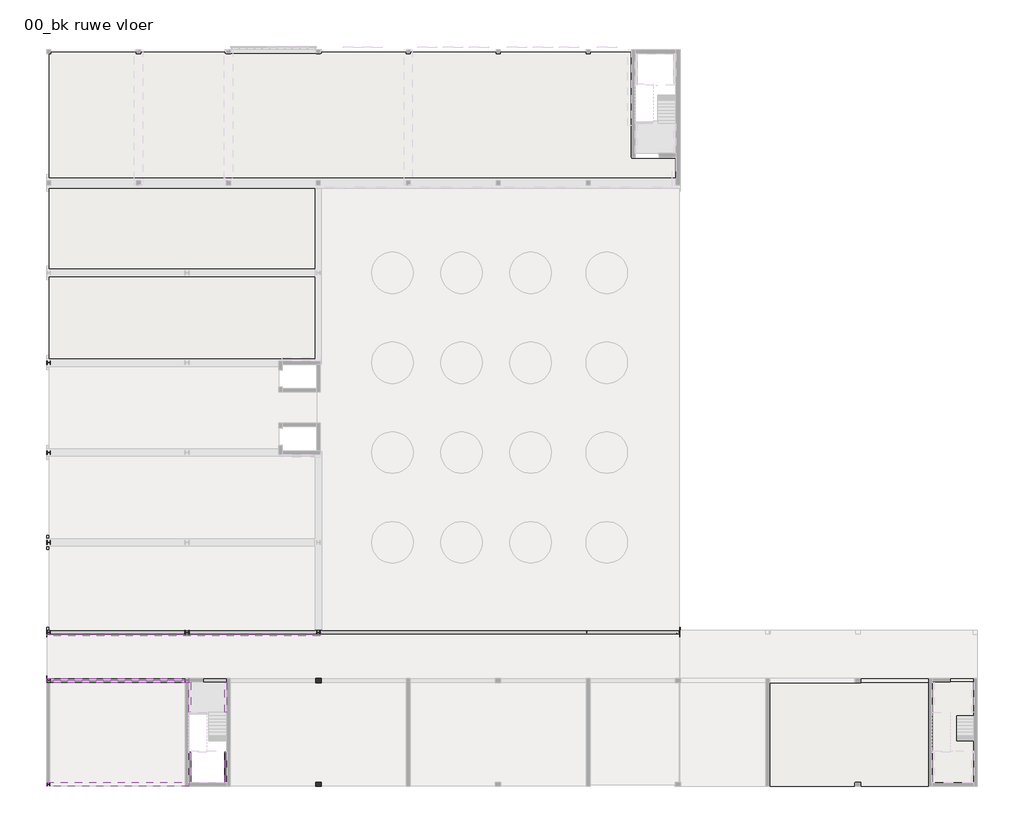
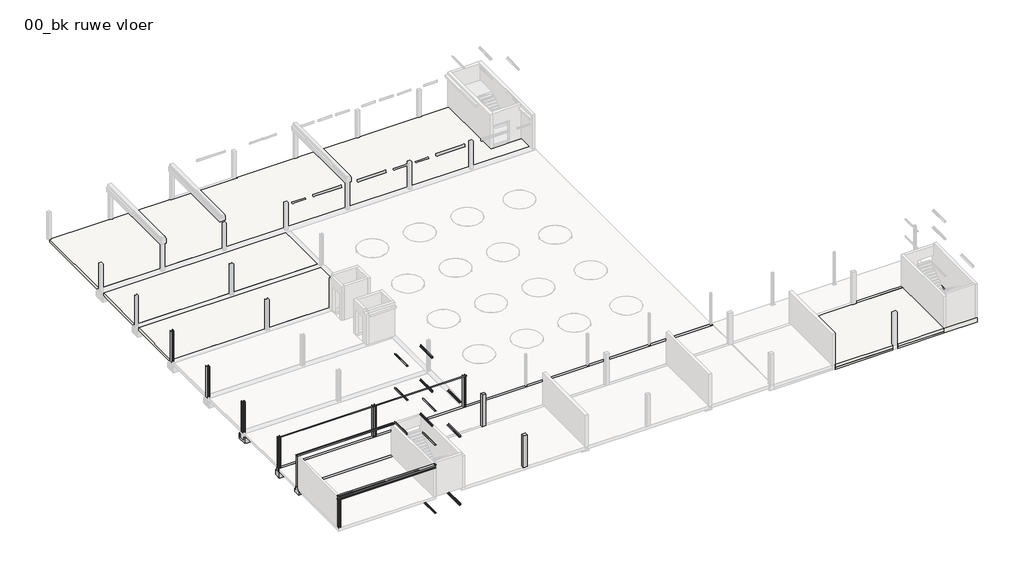
# One storey, part 4 of 6: 24 beams, 10 columns, 8 slabs.
# Revit data of these elements (continued)
# Type "NLRS_28_SF_LIB_stalen ligger stripstaal-AV-MMBS-SRP_gen_rsf : stalen ligger stripstaal RECT_gen__120x15" (continued)
#   NLRS_C_lengte [instance default] = 1500 mm
#   Length [instance default] = 1500 mm
#   bf = 120 mm
#   d = 15 mm
#   Structural Material = NLRS_h2_staal_gen_rsf
#   Keynote = ""
# Type "NLRS_28_SF_LIB_stalen ligger hoekprofiel gelijkzijdig-AV-MMBS-SRP_gen_rsf : stalen ligger gelijkzijdig hoekprofiel LEQU_gen__150x150x15"
#   Type IfcGUID = "2CEqVLPNH8KRN7ghwV3a1U"
#   IfcExportAs = "IfcBeamType"
#   Type Comments = "L150x150x15"
#   Model = " "
#   Manufacturer = " "
#   Fire Rating = " "
#   Description = "stalen ligger L150x150x15"
#   Assembly Code = "28.11"
#   vz = 107.5 mm
#   vy = 107.5 mm
#   tw = 15 mm
#   tf = 15 mm
#   ri = 8 mm
#   ra = 16 mm
#   d = 150 mm
#   bf = 150 mm
#   NLRS_C_lengte [instance default] = 1524 mm
#   Length [instance default] = 1524 mm
#   Structural Material = NLRS_h2_staal_gen_rsf
#   Keynote = ""
# Type "NLRS_28_SCO_TLB_stalen kolom HEA-BCPG-MMBS-SRP_gen_rsf : stalen kolom_gen__HEA 260"
#   Type IfcGUID = "2$hNzCXOT3YR8V$0CfyzGd"
#   IfcExportAs = "IfcColumnType"
#   IfcExportType = "COLUMN"
#   Type Comments = "HEA260"
#   Model = " "
#   Manufacturer = " "
#   Description = "stalen kolom HEA260"
#   Assembly Code = "28.11"
#   vz = 125 mm
#   vy = 130 mm
#   vpz = 125 mm
#   vpy = 130 mm
#   tw = 7.5 mm
#   tf = 12.5 mm
#   ra = 24 mm
#   d = 250 mm
#   bf = 260 mm
#   NLRS_C_lengte [instance default] = 2743.2 mm
#   Structural Material = NLRS_h2_staal_gen_rsf
#   Keynote = ""
# Type "NLRS_28_SCO_TLB_stalen kolom HEB-BCPG-MMBS-SRP_gen_rsf : stalen kolom_gen__HEB 300"
#   Type IfcGUID = "3C_b5Xdrv818Ti1jf59K4n"
#   IfcExportAs = "IfcColumnType"
#   IfcExportType = "COLUMN"
#   Type Comments = "HEB300"
#   Model = " "
#   Manufacturer = " "
#   Description = "stalen kolom HEB300"
#   Assembly Code = "28.11"
#   vz = 150 mm
#   vy = 150 mm
#   vpz = 150 mm
#   vpy = 150 mm
#   tw = 11 mm
#   tf = 19 mm
#   ra = 27 mm
#   d = 300 mm
#   bf = 300 mm
#   NLRS_C_lengte [instance default] = 2743.2 mm
#   Structural Material = NLRS_h2_staal_gen_rsf
#   Keynote = ""
# Type "NLRS_28_SCO_TLB_vierkante kolom beton ihwg-BCPG-MMBC-SRP_gen_rsf : vierkante kolom beton ihwg_gen__bxh 400x300"
#   Type IfcGUID = "2lw04Qbvr9TgC3fLWwYn2N"
#   IfcExportAs = "IfcColumnType"
#   IfcExportType = "COLUMN"
#   Type Comments = "400x300"
#   Model = "LOD300"
#   Description = "betonkolom ihwg 400x300"
#   Assembly Code = "28.11"
#   NLRS_C_lengte [instance default] = 2700 mm
#   NLRS_C_hoogte = 300 mm
#   NLRS_C_breedte = 400 mm
#   Structural Material = NLRS_f2_beton ihwg_gen_rsf
# Type "NLRS_28_SCO_TLB_stalen kolom HEA-BCPG-MMBS-SRP_gen_rsf : stalen kolom_gen__HEA 240"
#   Type IfcGUID = "2$hNzCXOT3YR8V$0CfyzVH"
#   IfcExportAs = "IfcColumnType"
#   IfcExportType = "COLUMN"
#   Type Comments = "HEA240"
#   Model = " "
#   Manufacturer = " "
#   Description = "stalen kolom HEA240"
#   Assembly Code = "28.11"
#   vz = 115 mm
#   vy = 120 mm
#   vpz = 115 mm
#   vpy = 120 mm
#   tw = 7.5 mm
#   tf = 12 mm
#   ra = 21 mm
#   d = 230 mm
#   bf = 240 mm
#   NLRS_C_lengte [instance default] = 2743.2 mm
#   Structural Material = NLRS_h2_staal_gen_rsf
#   Keynote = ""
# Type "NLRS_28_SCO_TLB_stalen kolom HEA-BCPG-MMBS-SRP_gen_rsf : stalen kolom_gen__HEA 200"
#   Type IfcGUID = "2$hNzCXOT3YR8V$0CfyzVT"
#   IfcExportAs = "IfcColumnType"
#   IfcExportType = "COLUMN"
#   Type Comments = "HEA200"
#   Model = " "
#   Manufacturer = " "
#   Description = "stalen kolom HEA200"
#   Assembly Code = "28.11"
#   vz = 95 mm
#   vy = 100 mm
#   vpz = 95 mm
#   vpy = 100 mm
#   tw = 6.5 mm
#   tf = 10 mm
#   ra = 18 mm
#   d = 190 mm
#   bf = 200 mm
#   NLRS_C_lengte [instance default] = 2743.2 mm
#   Structural Material = NLRS_h2_staal_gen_rsf
#   Keynote = ""
# Type "NLRS_23_FL_isolatieplaatvloer 320_gen_rsf"
#   Keynote = ""
#   Type IfcGUID = "0X0KViByb4JPBOa4XaNeBK"
#   Type Comments = "d=320mm"
#   Description = "prefab isolatieplaatvloer, vrijdragend"
#   Assembly Code = "23.21"
#   IfcExportAs = "IfcSlab"
#   Function = 0
#   Layers, outside or top first: 40 mm "NLRS_f2_beton prefab_gen_rsf" (function 1); 235 mm "NLRS_f2_beton prefab_gen_rsf" (function 1); 45 mm "NLRS_f2_beton prefab_gen_rsf" (function 1)
# Type "NLRS_23_FL_beton ihwg vloeraanstort 520_gen_rsf"
#   Keynote = ""
#   Type IfcGUID = "3aMdMHoe12P9KDGPyaIe$w"
#   Type Comments = "vloeraanstort d=520"
#   Description = "in het werk gestorte betonvloer, vrijdragend"
#   Assembly Code = "23.21"
#   IfcExportAs = "IfcSlab"
#   Function = 0
#   Layers, outside or top first: 520 mm "NLRS_f2_beton ihwg_gen_rsf" (function 1)
# Type "NLRS_23_FL_isolatie isolatieplaatvloer 200_gen_rsf"
#   Keynote = ""
#   Type IfcGUID = "3aMdMHoe12P9KDGPyaIfI8"
#   Type Comments = "d=200mm"
#   Description = "prefab isolatieplaatvloer, vrijdragend"
#   Assembly Code = "23.21"
#   IfcExportAs = "IfcSlab"
#   Function = 0
#   Layers, outside or top first: 200 mm "NLRS_n7_isolatie EPS_gen_rsf" (function 1)
# Element 1 (IfcBeam, "NLRS_28_SF_LIB_balk dubbele sponning beton prefab-CWV-MMBC-SRP_gen_rsf : balk beton prefab_gen__bxh 700x900 met inkassing bxh 200x320")
#   IfcGUID = "0AFZSao6j3uApvehgmz3cS"
#   NLRS_C_lengte = 45800 mm
#   IsExternal = yes
#   LoadBearing = yes
#   Phase Created = NLRS_nieuw
#   Materials on its faces: "NLRS_f2_beton prefab_gen_rsf"
# Element 2 (IfcBeam, "NLRS_28_SF_LIB_balkbodem beton prefab-CWV-MMBC-SRP_gen_rsf : balkbodem beton prefab_gen__bxhxdk 1000x580x200")
#   IfcGUID = "0X0KViByb4JPBOa4XaNgPp"
#   NLRS_C_lengte = 19200 mm
#   IsExternal = yes
#   LoadBearing = yes
#   Phase Created = NLRS_nieuw
#   Materials on its faces: "NLRS_f2_beton prefab_gen_rsf"
# Element 3 (IfcBeam, "NLRS_28_SF_LIB_balk dubbele sponning beton prefab-CWV-MMBC-SRP_gen_rsf : balk beton prefab_gen__bxh 700x700 met inkassing bxh 200x320")
#   IfcGUID = "1pBmRfcsbA7BE9s_rekBS$"
#   NLRS_C_lengte = 10150 mm
#   IsExternal = yes
#   LoadBearing = yes
#   Phase Created = NLRS_nieuw
#   Materials on its faces: "NLRS_f2_beton prefab_gen_rsf", "NLRS_f2_beton ihwg_gen_rsf"
# Element 4 (IfcBeam, "NLRS_28_SF_LIB_balk dubbele sponning beton prefab-CWV-MMBC-SRP_gen_rsf : balk beton prefab_gen__bxh 700x700 met inkassing bxh 200x320")
#   IfcGUID = "1pBmRfcsbA7BE9s_rekB42"
#   NLRS_C_lengte = 2875 mm
#   IsExternal = yes
#   LoadBearing = yes
#   Phase Created = NLRS_nieuw
#   Materials on its faces: "NLRS_f2_beton prefab_gen_rsf"
# Element 5 (IfcBeam, "NLRS_28_SF_LIB_stalen ligger HEB-AV-CWV-MMBS-SRP_gen_rsf : stalen ligger_gen__HEB 360")
#   IfcGUID = "00ECIG4lbEgBwDs3wwpaJg"
#   Comments = ""
#   NLRS_C_lengte = 10275 mm
#   IsExternal = no
#   LoadBearing = yes
#   Phase Created = NLRS_nieuw
#   Materials on its faces: "NLRS_h2_staal_gen_rsf"
# Element 6 (IfcBeam, "NLRS_28_SF_LIB_stalen ligger stripstaal-AV-MMBS-SRP_gen_rsf : stalen ligger stripstaal RECT_gen__140x15")
#   IfcGUID = "00ECIG4lbEgBwDs3wwpaJk"
#   Comments = ""
#   NLRS_C_lengte = 10275 mm
#   IsExternal = no
#   LoadBearing = yes
#   Phase Created = NLRS_nieuw
#   Materials on its faces: "NLRS_h2_staal_gen_rsf"
# Element 7 (IfcBeam, "NLRS_28_SF_LIB_stalen ligger stripstaal-AV-MMBS-SRP_gen_rsf : stalen ligger stripstaal RECT_gen__140x15")
#   IfcGUID = "00ECIG4lbEgBwDs3wwpaJi"
#   Comments = ""
#   NLRS_C_lengte = 10275 mm
#   IsExternal = no
#   LoadBearing = yes
#   Phase Created = NLRS_nieuw
#   Materials on its faces: "NLRS_h2_staal_gen_rsf"
# Element 8 (IfcBeam, "NLRS_28_SF_LIB_stalen ligger stripstaal-AV-MMBS-SRP_gen_rsf : stalen ligger stripstaal RECT_gen__120x15")
#   IfcGUID = "30fJl_yZvFzewSfsmFGxE0"
#   Comments = ""
#   NLRS_C_lengte = 19775 mm
#   IsExternal = no
#   LoadBearing = yes
#   Phase Created = NLRS_nieuw
#   Materials on its faces: "NLRS_h2_staal_gen_rsf"
# Element 9 (IfcBeam, "NLRS_28_SF_LIB_stalen ligger hoekprofiel gelijkzijdig-AV-MMBS-SRP_gen_rsf : stalen ligger gelijkzijdig hoekprofiel LEQU_gen__150x150x15")
#   IfcGUID = "2CEqVLPNH8KRN7ghwV3a5c"
#   NLRS_C_lengte = 2190 mm
#   IsExternal = no
#   LoadBearing = yes
#   Phase Created = NLRS_nieuw
#   Materials on its faces: "NLRS_h2_staal_gen_rsf"
# Element 10 (IfcBeam, "NLRS_28_SF_LIB_stalen ligger hoekprofiel gelijkzijdig-AV-MMBS-SRP_gen_rsf : stalen ligger gelijkzijdig hoekprofiel LEQU_gen__150x150x15")
#   IfcGUID = "2CEqVLPNH8KRN7ghwV3by5"
#   NLRS_C_lengte = 2190 mm
#   IsExternal = no
#   LoadBearing = yes
#   Phase Created = NLRS_nieuw
#   Materials on its faces: "NLRS_h2_staal_gen_rsf"
# Element 11 (IfcBeam, "NLRS_28_SF_LIB_stalen ligger hoekprofiel gelijkzijdig-AV-MMBS-SRP_gen_rsf : stalen ligger gelijkzijdig hoekprofiel LEQU_gen__150x150x15")
#   IfcGUID = "2CEqVLPNH8KRN7ghwV3by_"
#   NLRS_C_lengte = 2190 mm
#   IsExternal = no
#   LoadBearing = yes
#   Phase Created = NLRS_nieuw
#   Materials on its faces: "NLRS_h2_staal_gen_rsf"
# Element 12 (IfcBeam, "NLRS_28_SF_LIB_stalen ligger hoekprofiel gelijkzijdig-AV-MMBS-SRP_gen_rsf : stalen ligger gelijkzijdig hoekprofiel LEQU_gen__150x150x15")
#   IfcGUID = "2CEqVLPNH8KRN7ghwV3bzN"
#   NLRS_C_lengte = 2190 mm
#   IsExternal = no
#   LoadBearing = yes
#   Phase Created = NLRS_nieuw
#   Materials on its faces: "NLRS_h2_staal_gen_rsf"
# Element 13 (IfcBeam, "NLRS_28_SF_LIB_stalen ligger hoekprofiel gelijkzijdig-AV-MMBS-SRP_gen_rsf : stalen ligger gelijkzijdig hoekprofiel LEQU_gen__150x150x15")
#   IfcGUID = "2CEqVLPNH8KRN7ghwV3b_X"
#   NLRS_C_lengte = 2190 mm
#   IsExternal = no
#   LoadBearing = yes
#   Phase Created = NLRS_nieuw
#   Materials on its faces: "NLRS_h2_staal_gen_rsf"
# Element 14 (IfcBeam, "NLRS_28_SF_LIB_stalen ligger hoekprofiel gelijkzijdig-AV-MMBS-SRP_gen_rsf : stalen ligger gelijkzijdig hoekprofiel LEQU_gen__150x150x15")
#   IfcGUID = "2CEqVLPNH8KRN7ghwV3baI"
#   NLRS_C_lengte = 2190 mm
#   IsExternal = no
#   LoadBearing = yes
#   Phase Created = NLRS_nieuw
#   Materials on its faces: "NLRS_h2_staal_gen_rsf"
# Element 15 (IfcBeam, "NLRS_28_SF_LIB_stalen ligger hoekprofiel gelijkzijdig-AV-MMBS-SRP_gen_rsf : stalen ligger gelijkzijdig hoekprofiel LEQU_gen__150x150x15")
#   IfcGUID = "2CEqVLPNH8KRN7ghwV3baB"
#   NLRS_C_lengte = 2190 mm
#   IsExternal = no
#   LoadBearing = yes
#   Phase Created = NLRS_nieuw
#   Materials on its faces: "NLRS_h2_staal_gen_rsf"
# Element 16 (IfcBeam, "NLRS_28_SF_LIB_stalen ligger hoekprofiel gelijkzijdig-AV-MMBS-SRP_gen_rsf : stalen ligger gelijkzijdig hoekprofiel LEQU_gen__150x150x15")
#   IfcGUID = "2CEqVLPNH8KRN7ghwV3bai"
#   NLRS_C_lengte = 2190 mm
#   IsExternal = no
#   LoadBearing = yes
#   Phase Created = NLRS_nieuw
#   Materials on its faces: "NLRS_h2_staal_gen_rsf"
# Element 17 (IfcBeam, "NLRS_28_SF_LIB_stalen ligger hoekprofiel gelijkzijdig-AV-MMBS-SRP_gen_rsf : stalen ligger gelijkzijdig hoekprofiel LEQU_gen__150x150x15")
#   IfcGUID = "2CEqVLPNH8KRN7ghwV3bxp"
#   NLRS_C_lengte = 2190 mm
#   IsExternal = no
#   LoadBearing = yes
#   Phase Created = NLRS_nieuw
#   Materials on its faces: "NLRS_h2_staal_gen_rsf"
# Element 18 (IfcBeam, "NLRS_28_SF_LIB_stalen ligger hoekprofiel gelijkzijdig-AV-MMBS-SRP_gen_rsf : stalen ligger gelijkzijdig hoekprofiel LEQU_gen__150x150x15")
#   IfcGUID = "2CEqVLPNH8KRN7ghwV3by0"
#   NLRS_C_lengte = 2190 mm
#   IsExternal = no
#   LoadBearing = yes
#   Phase Created = NLRS_nieuw
#   Materials on its faces: "NLRS_h2_staal_gen_rsf"
# Element 19 (IfcBeam, "NLRS_28_SF_LIB_stalen ligger hoekprofiel gelijkzijdig-AV-MMBS-SRP_gen_rsf : stalen ligger gelijkzijdig hoekprofiel LEQU_gen__150x150x15")
#   IfcGUID = "2CEqVLPNH8KRN7ghwV3byv"
#   NLRS_C_lengte = 2190 mm
#   IsExternal = no
#   LoadBearing = yes
#   Phase Created = NLRS_nieuw
#   Materials on its faces: "NLRS_h2_staal_gen_rsf"
# Element 20 (IfcBeam, "NLRS_28_SF_LIB_stalen ligger hoekprofiel gelijkzijdig-AV-MMBS-SRP_gen_rsf : stalen ligger gelijkzijdig hoekprofiel LEQU_gen__150x150x15")
#   IfcGUID = "2CEqVLPNH8KRN7ghwV3bzI"
#   NLRS_C_lengte = 2190 mm
#   IsExternal = no
#   LoadBearing = yes
#   Phase Created = NLRS_nieuw
#   Materials on its faces: "NLRS_h2_staal_gen_rsf"
# Element 21 (IfcBeam, "NLRS_28_SF_LIB_stalen ligger hoekprofiel gelijkzijdig-AV-MMBS-SRP_gen_rsf : stalen ligger gelijkzijdig hoekprofiel LEQU_gen__150x150x15")
#   IfcGUID = "2CEqVLPNH8KRN7ghwV3b_i"
#   NLRS_C_lengte = 2190 mm
#   IsExternal = no
#   LoadBearing = yes
#   Phase Created = NLRS_nieuw
#   Materials on its faces: "NLRS_h2_staal_gen_rsf"
# Element 22 (IfcBeam, "NLRS_28_SF_LIB_stalen ligger hoekprofiel gelijkzijdig-AV-MMBS-SRP_gen_rsf : stalen ligger gelijkzijdig hoekprofiel LEQU_gen__150x150x15")
#   IfcGUID = "2CEqVLPNH8KRN7ghwV3baS"
#   NLRS_C_lengte = 2190 mm
#   IsExternal = no
#   LoadBearing = yes
#   Phase Created = NLRS_nieuw
#   Materials on its faces: "NLRS_h2_staal_gen_rsf"
# Element 23 (IfcBeam, "NLRS_28_SF_LIB_stalen ligger hoekprofiel gelijkzijdig-AV-MMBS-SRP_gen_rsf : stalen ligger gelijkzijdig hoekprofiel LEQU_gen__150x150x15")
#   IfcGUID = "2CEqVLPNH8KRN7ghwV3bar"
#   NLRS_C_lengte = 2190 mm
#   IsExternal = no
#   LoadBearing = yes
#   Phase Created = NLRS_nieuw
#   Materials on its faces: "NLRS_h2_staal_gen_rsf"
# Element 24 (IfcBeam, "NLRS_28_SF_LIB_stalen ligger hoekprofiel gelijkzijdig-AV-MMBS-SRP_gen_rsf : stalen ligger gelijkzijdig hoekprofiel LEQU_gen__150x150x15")
#   IfcGUID = "2CEqVLPNH8KRN7ghwV3bak"
#   NLRS_C_lengte = 2190 mm
#   IsExternal = no
#   LoadBearing = yes
#   Phase Created = NLRS_nieuw
#   Materials on its faces: "NLRS_h2_staal_gen_rsf"
# Element 25 (IfcColumn, "NLRS_28_SCO_TLB_stalen kolom HEA-BCPG-MMBS-SRP_gen_rsf : stalen kolom_gen__HEA 260")
#   IfcGUID = "2$hNzCXOT3YR8V$0Cfyz77"
#   Comments = ""
#   IsExternal = no
#   LoadBearing = yes
#   Phase Created = NLRS_nieuw
#   Materials on its faces: "NLRS_h2_staal_gen_rsf"
# Element 26 (IfcColumn, "NLRS_28_SCO_TLB_stalen kolom HEA-BCPG-MMBS-SRP_gen_rsf : stalen kolom_gen__HEA 260")
#   IfcGUID = "2$hNzCXOT3YR8V$0Cfyz53"
#   Comments = ""
#   IsExternal = no
#   LoadBearing = yes
#   Phase Created = NLRS_nieuw
#   Materials on its faces: "NLRS_h2_staal_gen_rsf"
# Element 27 (IfcColumn, "NLRS_28_SCO_TLB_stalen kolom HEA-BCPG-MMBS-SRP_gen_rsf : stalen kolom_gen__HEA 260")
#   IfcGUID = "2$hNzCXOT3YR8V$0Cfyz3A"
#   Comments = ""
#   IsExternal = no
#   LoadBearing = yes
#   Phase Created = NLRS_nieuw
#   Materials on its faces: "NLRS_h2_staal_gen_rsf"
# Element 28 (IfcColumn, "NLRS_28_SCO_TLB_stalen kolom HEA-BCPG-MMBS-SRP_gen_rsf : stalen kolom_gen__HEA 260")
#   IfcGUID = "2$hNzCXOT3YR8V$0Cfyz25"
#   Comments = ""
#   IsExternal = no
#   LoadBearing = yes
#   Phase Created = NLRS_nieuw
#   Materials on its faces: "NLRS_h2_staal_gen_rsf"
# Element 29 (IfcColumn, "NLRS_28_SCO_TLB_stalen kolom HEB-BCPG-MMBS-SRP_gen_rsf : stalen kolom_gen__HEB 300")
#   IfcGUID = "2GRbcre991teoKeCLB8Lxz"
#   Comments = ""
#   IsExternal = no
#   LoadBearing = yes
#   Phase Created = NLRS_nieuw
#   Materials on its faces: "NLRS_h2_staal_gen_rsf"
# Element 30 (IfcColumn, "NLRS_28_SCO_TLB_stalen kolom HEA-BCPG-MMBS-SRP_gen_rsf : stalen kolom_gen__HEA 260")
#   IfcGUID = "2GRbcre991teoKeCLB8Lws"
#   Comments = ""
#   IsExternal = no
#   LoadBearing = yes
#   Phase Created = NLRS_nieuw
#   Materials on its faces: "NLRS_h2_staal_gen_rsf"
# Element 31 (IfcColumn, "NLRS_28_SCO_TLB_vierkante kolom beton ihwg-BCPG-MMBC-SRP_gen_rsf : vierkante kolom beton ihwg_gen__bxh 400x300")
#   IfcGUID = "2lw04Qbvr9TgC3fLWwYnCj"
#   IsExternal = no
#   LoadBearing = yes
#   Phase Created = NLRS_nieuw
#   Materials on its faces: "NLRS_f2_beton ihwg_gen_rsf"
# Element 32 (IfcColumn, "NLRS_28_SCO_TLB_vierkante kolom beton ihwg-BCPG-MMBC-SRP_gen_rsf : vierkante kolom beton ihwg_gen__bxh 400x300")
#   IfcGUID = "2lw04Qbvr9TgC3fLWwYn7v"
#   IsExternal = no
#   LoadBearing = yes
#   Phase Created = NLRS_nieuw
#   Materials on its faces: "NLRS_f2_beton ihwg_gen_rsf"
# Element 33 (IfcColumn, "NLRS_28_SCO_TLB_stalen kolom HEA-BCPG-MMBS-SRP_gen_rsf : stalen kolom_gen__HEA 240")
#   IfcGUID = "00ECIG4lbEgBwDs3wwpb$e"
#   Comments = ""
#   IsExternal = no
#   LoadBearing = yes
#   Phase Created = NLRS_nieuw
#   Materials on its faces: "NLRS_h2_staal_gen_rsf"
# Element 34 (IfcColumn, "NLRS_28_SCO_TLB_stalen kolom HEA-BCPG-MMBS-SRP_gen_rsf : stalen kolom_gen__HEA 200")
#   IfcGUID = "00ECIG4lbEgBwDs3wwpbsp"
#   Comments = ""
#   IsExternal = no
#   LoadBearing = yes
#   Phase Created = NLRS_nieuw
#   Materials on its faces: "NLRS_h2_staal_gen_rsf"
# Element 35 (IfcSlab, "NLRS_23_FL_isolatieplaatvloer 320_gen_rsf")
#   IfcGUID = "2bNskL0kfByRmbY5G6IfIf"
#   built-in parameter 1001955 = 1.5708 (stored number, unit not read)
#   Height Offset From Level = 0 mm
#   built-in parameter 1001954 = 1
#   IsExternal = yes
#   LoadBearing = yes
#   Phase Created = NLRS_nieuw
#   Materials on its faces: "NLRS_f2_beton prefab_gen_rsf"
# Element 36 (IfcSlab, "NLRS_23_FL_isolatieplaatvloer 320_gen_rsf")
#   IfcGUID = "2bNskL0kfByRmbY5G6IfNQ"
#   built-in parameter 1001955 = 1.5708 (stored number, unit not read)
#   Height Offset From Level = 0 mm
#   built-in parameter 1001954 = 1
#   IsExternal = yes
#   LoadBearing = yes
#   Phase Created = NLRS_nieuw
#   Materials on its faces: "NLRS_f2_beton prefab_gen_rsf"
# Element 37 (IfcSlab, "NLRS_23_FL_isolatieplaatvloer 320_gen_rsf")
#   IfcGUID = "1E6t7WhRf97hJGfj3Bm3pQ"
#   Comments = ""
#   built-in parameter 1001955 = -1.5708 (stored number, unit not read)
#   Height Offset From Level = 0 mm
#   built-in parameter 1001954 = 1
#   IsExternal = yes
#   LoadBearing = yes
#   Phase Created = NLRS_nieuw
#   Materials on its faces: "NLRS_f2_beton prefab_gen_rsf"
# Element 38 (IfcSlab, "NLRS_23_FL_isolatieplaatvloer 320_gen_rsf")
#   IfcGUID = "2gNlyDOFb5qwP_T4qK0dKx"
#   Comments = ""
#   built-in parameter 1001955 = -1.5708 (stored number, unit not read)
#   Height Offset From Level = 0 mm
#   built-in parameter 1001954 = 1
#   IsExternal = yes
#   LoadBearing = yes
#   Phase Created = NLRS_nieuw
#   Materials on its faces: "NLRS_f2_beton prefab_gen_rsf"
# Element 39 (IfcSlab, "NLRS_23_FL_isolatieplaatvloer 320_gen_rsf")
#   IfcGUID = "0H0z87ABnEyOuaeN1efimG"
#   Comments = ""
#   built-in parameter 1001955 = 1.5708 (stored number, unit not read)
#   Height Offset From Level = 0 mm
#   built-in parameter 1001954 = 1
#   IsExternal = yes
#   LoadBearing = yes
#   Phase Created = NLRS_nieuw
#   Materials on its faces: "NLRS_f2_beton prefab_gen_rsf"
# Element 40 (IfcSlab, "NLRS_23_FL_beton ihwg vloeraanstort 520_gen_rsf")
#   IfcGUID = "3aMdMHoe12P9KDGPyaIeY6"
#   Height Offset From Level = 0 mm
#   built-in parameter 1001954 = 1
#   IsExternal = yes
#   LoadBearing = yes
#   Phase Created = NLRS_nieuw
#   Materials on its faces: "NLRS_f2_beton ihwg_gen_rsf"
# Element 41 (IfcSlab, "NLRS_23_FL_isolatie isolatieplaatvloer 200_gen_rsf")
#   IfcGUID = "3aMdMHoe12P9KDGPyaIfHv"
#   built-in parameter 1001955 = 1.5708 (stored number, unit not read)
#   Height Offset From Level = -320 mm
#   built-in parameter 1001954 = 1
#   IsExternal = yes
#   LoadBearing = yes
#   Phase Created = NLRS_nieuw
#   Materials on its faces: "NLRS_n7_isolatie EPS_gen_rsf"
# Element 42 (IfcSlab, "NLRS_23_FL_isolatie isolatieplaatvloer 200_gen_rsf")
#   IfcGUID = "3aMdMHoe12P9KDGPyaIfLI"
#   built-in parameter 1001955 = 1.5708 (stored number, unit not read)
#   Height Offset From Level = -320 mm
#   built-in parameter 1001954 = 1
#   IsExternal = yes
#   LoadBearing = yes
#   Phase Created = NLRS_nieuw
#   Materials on its faces: "NLRS_n7_isolatie EPS_gen_rsf"
# Materials
#   "NLRS_f2_beton prefab_gen_rsf": class "F - Niet gebakken kunststeen", colour RGB 129 133 118, transparency 0, Keynote = "f2", Manufacturer = "Revit Standards Foundation", URL = "www.revitstandards.org", Description = "beton prefab", Cost = 0
#   "NLRS_h2_staal_gen_rsf": class "H - Metaal", colour RGB 189 187 185, transparency 0, Keynote = "h2", Manufacturer = "Revit Standards Foundation", URL = "www.revitstandards.org", Description = "staal", Cost = 0
#   "NLRS_f2_beton ihwg_gen_rsf": class "F - Niet gebakken kunststeen", colour RGB 129 133 118, transparency 0, Keynote = "f2", Manufacturer = "Revit Standards Foundation", URL = "www.revitstandards.org", Description = "beton ihwg", Cost = 0
#   "NLRS_n7_isolatie EPS_gen_rsf": class "N - Kunststoffen, rubbers", colour RGB 200 200 140, transparency 0, Keynote = "n7", Manufacturer = "Revit Standards Foundation", URL = "www.revitstandards.org", Description = "isolatie EPS", Cost = 0
